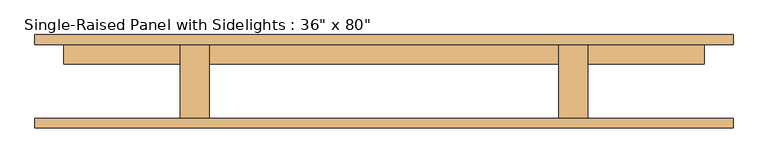
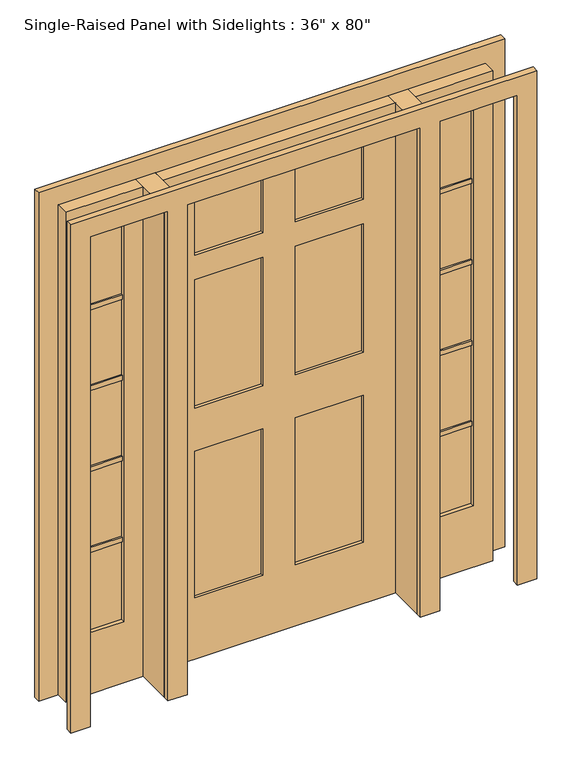
"""IFC4 building model written with IfcOpenShell, lengths in millimetres: door geometry."""

from ifc_helpers import new_model, si_unit, frame, origin, origin_with_axes, place, context, project, spatial, polyline, outline, extrude, source, transform, mapped, element, save


def door_f5e23370(model_context):
    return source(origin(), model_context, "Body", "SweptSolid", [
        extrude(outline(polyline([(762.0, 55.5625), (609.6, 55.5625), (609.6, 87.3125), (762.0, 87.3125), (762.0, 55.5625)])), frame((0.0, 0.0, 579.755), z_axis=(0.0, 0.0, 1.0), x_axis=(1.0, 0.0, 0.0)), (0.0, 0.0, 1.0), 19.05),
        extrude(outline(polyline([(762.0, 55.5625), (609.6, 55.5625), (609.6, 87.3125), (762.0, 87.3125), (762.0, 55.5625)])), frame((0.0, 0.0, 915.035), z_axis=(0.0, 0.0, 1.0), x_axis=(1.0, 0.0, 0.0)), (0.0, 0.0, 1.0), 19.05),
        extrude(outline(polyline([(762.0, 55.5625), (609.6, 55.5625), (609.6, 87.3125), (762.0, 87.3125), (762.0, 55.5625)])), frame((0.0, 0.0, 1250.315), z_axis=(0.0, 0.0, 1.0), x_axis=(1.0, 0.0, 0.0)), (0.0, 0.0, 1.0), 19.05),
        extrude(outline(polyline([(762.0, 55.5625), (609.6, 55.5625), (609.6, 87.3125), (762.0, 87.3125), (762.0, 55.5625)])), frame((0.0, 0.0, 1585.595), z_axis=(0.0, 0.0, 1.0), x_axis=(1.0, 0.0, 0.0)), (0.0, 0.0, 1.0), 19.05),
        extrude(outline(polyline([(-609.6, 55.5625), (-762.0, 55.5625), (-762.0, 87.3125), (-609.6, 87.3125), (-609.6, 55.5625)])), frame((0.0, 0.0, 1585.595), z_axis=(0.0, 0.0, 1.0), x_axis=(1.0, 0.0, 0.0)), (0.0, 0.0, 1.0), 19.05),
        extrude(outline(polyline([(-609.6, 55.5625), (-762.0, 55.5625), (-762.0, 87.3125), (-609.6, 87.3125), (-609.6, 55.5625)])), frame((0.0, 0.0, 1250.315), z_axis=(0.0, 0.0, 1.0), x_axis=(1.0, 0.0, 0.0)), (0.0, 0.0, 1.0), 19.05),
        extrude(outline(polyline([(-609.6, 55.5625), (-762.0, 55.5625), (-762.0, 87.3125), (-609.6, 87.3125), (-609.6, 55.5625)])), frame((0.0, 0.0, 915.035), z_axis=(0.0, 0.0, 1.0), x_axis=(1.0, 0.0, 0.0)), (0.0, 0.0, 1.0), 19.05),
        extrude(outline(polyline([(-609.6, 55.5625), (-762.0, 55.5625), (-762.0, 87.3125), (-609.6, 87.3125), (-609.6, 55.5625)])), frame((0.0, 0.0, 579.755), z_axis=(0.0, 0.0, 1.0), x_axis=(1.0, 0.0, 0.0)), (0.0, 0.0, 1.0), 19.05),
        extrude(outline(polyline([(762.0, 61.9125), (609.6, 61.9125), (609.6, 80.9625), (762.0, 80.9625), (762.0, 61.9125)])), frame((0.0, 0.0, 254.0), z_axis=(0.0, 0.0, 1.0), x_axis=(1.0, 0.0, 0.0)), (0.0, 0.0, 1.0), 1676.4),
        extrude(outline(polyline([(-609.6, 61.9125), (-762.0, 61.9125), (-762.0, 80.9625), (-609.6, 80.9625), (-609.6, 61.9125)])), frame((0.0, 0.0, 254.0), z_axis=(0.0, 0.0, 1.0), x_axis=(1.0, 0.0, 0.0)), (0.0, 0.0, 1.0), 1676.4),
        extrude(outline(polyline([(-457.2, -96.8375), (-533.4, -96.8375), (-533.4, 96.8375), (-457.2, 96.8375), (-457.2, -96.8375)])), origin_with_axes(), (0.0, 0.0, 1.0), 2032.0),
        extrude(outline(polyline([(533.4, -96.8375), (457.2, -96.8375), (457.2, 96.8375), (533.4, 96.8375), (533.4, -96.8375)])), origin_with_axes(), (0.0, 0.0, 1.0), 2032.0),
        extrude(outline(polyline([(2032.0, -533.4), (2032.0, -838.2), (0.0, -838.2), (0.0, -533.4), (2032.0, -533.4)]), holes=[polyline([(1930.4, -609.6), (254.0, -609.6), (254.0, -762.0), (1930.4, -762.0), (1930.4, -609.6)])]), frame((0.0, 46.0375, 0.0), z_axis=(0.0, 1.0, 0.0), x_axis=(0.0, 0.0, 1.0)), (0.0, 0.0, 1.0), 50.8),
        extrude(outline(polyline([(0.0, 533.4), (0.0, 838.2), (2032.0, 838.2), (2032.0, 533.4), (0.0, 533.4)]), holes=[polyline([(1930.4, 762.0), (254.0, 762.0), (254.0, 609.6), (1930.4, 609.6), (1930.4, 762.0)])]), frame((0.0, 46.0375, 0.0), z_axis=(0.0, 1.0, 0.0), x_axis=(0.0, 0.0, 1.0)), (0.0, 0.0, 1.0), 50.8),
        extrude(outline(polyline([(0.0, -914.4), (0.0, -838.2), (2032.0, -838.2), (2032.0, -533.4), (0.0, -533.4), (0.0, -457.2), (2032.0, -457.2), (2032.0, 457.2), (0.0, 457.2), (0.0, 533.4), (2032.0, 533.4), (2032.0, 838.2), (0.0, 838.2), (0.0, 914.4), (2108.2, 914.4), (2108.2, -914.4), (0.0, -914.4)])), frame((0.0, -122.2375, 0.0), z_axis=(0.0, 1.0, 0.0), x_axis=(0.0, 0.0, 1.0)), (0.0, 0.0, 1.0), 25.4),
        extrude(outline(polyline([(0.0, 914.4), (2108.2, 914.4), (2108.2, -914.4), (0.0, -914.4), (0.0, -838.2), (2032.0, -838.2), (2032.0, -533.4), (0.0, -533.4), (0.0, -457.2), (2032.0, -457.2), (2032.0, 457.2), (0.0, 457.2), (0.0, 533.4), (2032.0, 533.4), (2032.0, 838.2), (0.0, 838.2), (0.0, 914.4)])), frame((0.0, 96.8375, 0.0), z_axis=(0.0, 1.0, 0.0), x_axis=(0.0, 0.0, 1.0)), (0.0, 0.0, 1.0), 25.4),
        extrude(outline(polyline([(-63.5, 58.7375), (-330.2, 58.7375), (-330.2, 84.1375), (-63.5, 84.1375), (-63.5, 58.7375)])), frame((0.0, 0.0, 1676.4), z_axis=(0.0, 0.0, 1.0), x_axis=(1.0, 0.0, 0.0)), (0.0, 0.0, 1.0), 254.0),
        extrude(outline(polyline([(330.2, 58.7375), (63.5, 58.7375), (63.5, 84.1375), (330.2, 84.1375), (330.2, 58.7375)])), frame((0.0, 0.0, 1676.4), z_axis=(0.0, 0.0, 1.0), x_axis=(1.0, 0.0, 0.0)), (0.0, 0.0, 1.0), 254.0),
        extrude(outline(polyline([(-63.5, 58.7375), (-330.2, 58.7375), (-330.2, 84.1375), (-63.5, 84.1375), (-63.5, 58.7375)])), frame((0.0, 0.0, 1041.4), z_axis=(0.0, 0.0, 1.0), x_axis=(1.0, 0.0, 0.0)), (0.0, 0.0, 1.0), 533.4),
        extrude(outline(polyline([(330.2, 58.7375), (63.5, 58.7375), (63.5, 84.1375), (330.2, 84.1375), (330.2, 58.7375)])), frame((0.0, 0.0, 1041.4), z_axis=(0.0, 0.0, 1.0), x_axis=(1.0, 0.0, 0.0)), (0.0, 0.0, 1.0), 533.4),
        extrude(outline(polyline([(-63.5, 58.7375), (-330.2, 58.7375), (-330.2, 84.1375), (-63.5, 84.1375), (-63.5, 58.7375)])), frame((0.0, 0.0, 254.0), z_axis=(0.0, 0.0, 1.0), x_axis=(1.0, 0.0, 0.0)), (0.0, 0.0, 1.0), 609.6),
        extrude(outline(polyline([(330.2, 58.7375), (63.5, 58.7375), (63.5, 84.1375), (330.2, 84.1375), (330.2, 58.7375)])), frame((0.0, 0.0, 254.0), z_axis=(0.0, 0.0, 1.0), x_axis=(1.0, 0.0, 0.0)), (0.0, 0.0, 1.0), 609.6),
        extrude(outline(polyline([(2032.0, 457.2), (2032.0, -457.2), (0.0, -457.2), (0.0, 457.2), (2032.0, 457.2)]), holes=[polyline([(1930.4, -63.5), (1676.4, -63.5), (1676.4, -330.2), (1930.4, -330.2), (1930.4, -63.5)]), polyline([(1930.4, 330.2), (1676.4, 330.2), (1676.4, 63.5), (1930.4, 63.5), (1930.4, 330.2)]), polyline([(1574.8, -63.5), (1041.4, -63.5), (1041.4, -330.2), (1574.8, -330.2), (1574.8, -63.5)]), polyline([(1574.8, 330.2), (1041.4, 330.2), (1041.4, 63.5), (1574.8, 63.5), (1574.8, 330.2)]), polyline([(863.6, -63.5), (254.0, -63.5), (254.0, -330.2), (863.6, -330.2), (863.6, -63.5)]), polyline([(863.6, 330.2), (254.0, 330.2), (254.0, 63.5), (863.6, 63.5), (863.6, 330.2)])]), frame((0.0, 46.0375, 0.0), z_axis=(0.0, 1.0, 0.0), x_axis=(0.0, 0.0, 1.0)), (0.0, 0.0, 1.0), 50.8),
    ])


if __name__ == "__main__":
    model = new_model("IFC4")
    model_context = context("Model", 3, world=origin())
    ifc_project = project(units=[si_unit("LENGTHUNIT", "METRE", prefix="MILLI")], contexts=[model_context])
    site = spatial("IfcSite", under=ifc_project)
    building = spatial("IfcBuilding", under=site)
    placement = place(None, origin())
    door_shape = door_f5e23370(model_context)
    element("IfcDoor", 1, ObjectType="Single-Raised Panel with Sidelights : 36\" x 80\"", at=placement, inside=building, context=model_context, shape_type="MappedRepresentation", body=[
        mapped(door_shape, transform((0.0, 0.0, 0.0), x_axis=(1.0, 0.0, 0.0), y_axis=(0.0, 1.0, 0.0), z_axis=(0.0, 0.0, 1.0))),
    ])
    save(model, "model.ifc")

# Revit data of these elements
# Type "Single-Raised Panel with Sidelights : 36\" x 80\""
#   Type Mark = "47"
#   Assembly Code = "C1020"
#   Thickness = 0' - 2"
#   Height = 6' - 8"
#   Rail Width - Base = 0' - 10"
#   Rail Width - Center = 0' - 7"
#   Rail Width - Top = 0' - 4"
#   Sidelight Width = 1' - 0"
#   Stile Width = 0' - 5"
#   Trim Projection Ext = 0' - 1"
#   Trim Projection Int = 0' - 1"
#   Trim Width = 0' - 3"
#   Width = 3' - 0"
#   Define Thermal Properties by = 0
#   Function = 1
#   Door Material = Door - Panel
#   Frame Material = Door - Frame
#   Wall Closure = (empty or 0)
# Element 1 (IfcDoor, "Single-Raised Panel with Sidelights : 36\" x 80\"")
#   Materials on its faces: "Door - Panel", "Door - Frame", "Glass"
# Materials
#   "Door - Panel": class "Wood", colour RGB 227 170 128, transparency 0, Cost = 0
#   "Door - Frame": class "Miscellaneous", colour RGB 153 76 43, transparency 0, Cost = 0
#   "Glass": class "Glass", colour RGB 236 240 239, transparency 0.5, Description = "Soda Lime Glass", Cost = 0
